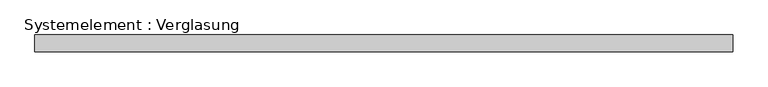
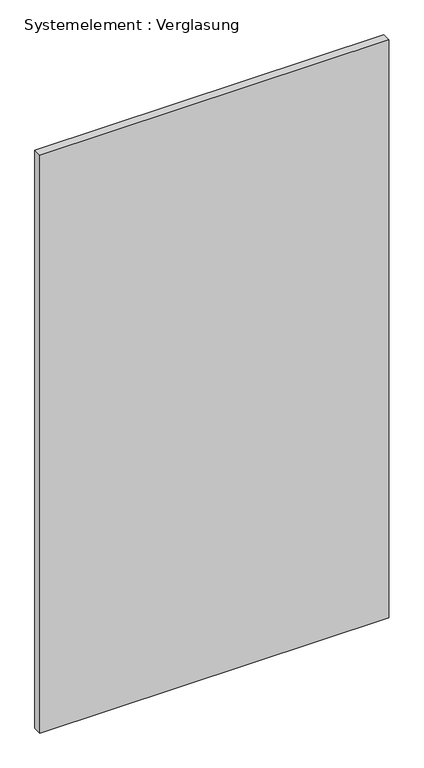
"""IFC4 building model written with IfcOpenShell, lengths in millimetres: plate geometry, Systemelement : Verglasung."""

import ifcopenshell
import ifcopenshell.guid

model = None  # the IFC model being written
_history = None  # IfcOwnerHistory: only IFC2X3 demands one
_inside = {}  # id of a spatial element -> (the spatial element, [elements in it])
_under = {}  # id of a project, library or spatial element -> (it, [spatial elements below it])
_declared = {}  # id of a project -> (the project, [libraries it declares])
_typed = {}  # id of a type object -> (the type object, [elements of that type])
_made_of = {}  # id of a material, layer set ... -> (it, [elements and type objects made of it])


def new_model(schema):
    """Start an empty IFC model of exactly this schema.

    Asked for "IFC4X3", IfcOpenShell would pick the latest addendum, in which some entities
    have other attributes; the version numbers below select the first issue.
    IFC2X3 requires an IfcOwnerHistory on every rooted entity: one is made here for all.
    """
    global model, _history
    if schema == "IFC4X3":
        model = ifcopenshell.file(schema_version=(4, 3, 0, 0))
    else:
        model = ifcopenshell.file(schema=schema)
    _inside.clear()
    _under.clear()
    _declared.clear()
    _typed.clear()
    _made_of.clear()
    _history = None
    if model.schema == "IFC2X3":
        org = make("IfcOrganization", Name="unknown")
        user = make(
            "IfcPersonAndOrganization",
            ThePerson=make("IfcPerson", FamilyName="unknown"),
            TheOrganization=org,
        )
        app = make(
            "IfcApplication",
            ApplicationDeveloper=org,
            Version="unknown",
            ApplicationFullName="unknown",
            ApplicationIdentifier="unknown",
        )
        _history = make(
            "IfcOwnerHistory",
            OwningUser=user,
            OwningApplication=app,
            ChangeAction="ADDED",
            CreationDate=0,
        )
    return model


def make(cls, **values):
    """One entity of the class cls with the attributes given. An attribute that is None is left unset."""
    return model.create_entity(
        cls, **{name: value for name, value in values.items() if value is not None}
    )


def rooted(cls, **values):
    """An entity with a GlobalId (a new one), such as an element, a storey or a relation."""
    return make(cls, GlobalId=ifcopenshell.guid.new(), OwnerHistory=_history, **values)


def si_unit(unit_type, name, prefix=None):
    """IfcSIUnit, for example si_unit("LENGTHUNIT", "METRE", prefix="MILLI")."""
    return make("IfcSIUnit", UnitType=unit_type, Prefix=prefix, Name=name)


def assignment(units):
    """IfcUnitAssignment: the units of a project."""
    return None if units is None else make("IfcUnitAssignment", Units=units)


def point(xyz):
    """IfcCartesianPoint."""
    return None if xyz is None else make("IfcCartesianPoint", Coordinates=xyz)


def direction(xyz):
    """IfcDirection."""
    return None if xyz is None else make("IfcDirection", DirectionRatios=xyz)


def frame(location, z_axis=None, x_axis=None):
    """IfcAxis2Placement3D, a coordinate frame: its origin and axes. An axis left out is left unset."""
    return make(
        "IfcAxis2Placement3D",
        Location=point(location),
        Axis=direction(z_axis),
        RefDirection=direction(x_axis),
    )


def origin():
    """The frame at (0, 0, 0) with its axes left unset."""
    return frame((0.0, 0.0, 0.0))


def origin_with_axes():
    """The frame at (0, 0, 0) with the z axis (0, 0, 1) and the x axis (1, 0, 0) written out."""
    return frame((0.0, 0.0, 0.0), z_axis=(0.0, 0.0, 1.0), x_axis=(1.0, 0.0, 0.0))


def place(relative_to, where):
    """IfcLocalPlacement: puts the frame where relative to a parent placement (None: the world)."""
    return make(
        "IfcLocalPlacement", PlacementRelTo=relative_to, RelativePlacement=where
    )


def context(
    kind, dimensions, precision=None, world=None, true_north=None, identifier=None
):
    """IfcGeometricRepresentationContext, for example the 3D "Model" context."""
    return make(
        "IfcGeometricRepresentationContext",
        ContextIdentifier=identifier,
        ContextType=kind,
        CoordinateSpaceDimension=dimensions,
        Precision=precision,
        WorldCoordinateSystem=world,
        TrueNorth=true_north,
    )


def project(units=None, contexts=None):
    """IfcProject with its units and contexts."""
    return rooted(
        "IfcProject",
        Name="project",
        RepresentationContexts=contexts,
        UnitsInContext=assignment(units),
    )


def spatial(cls, under=None, at=None, **own):
    """A site, building, storey or space (cls), placed at a placement, below another one or the project."""
    s = rooted(cls, ObjectPlacement=at, **own)
    if under is not None:
        _under.setdefault(under.id(), (under, []))[1].append(s)
    return s


def polyline(points):
    """IfcPolyline through the points."""
    return make("IfcPolyline", Points=[point(p) for p in points])


def outline(outer, holes=None, kind="AREA"):
    """IfcArbitraryClosedProfileDef: a profile drawn as a closed curve; with holes, ...WithVoids."""
    if holes is None:
        return make("IfcArbitraryClosedProfileDef", ProfileType=kind, OuterCurve=outer)
    return make(
        "IfcArbitraryProfileDefWithVoids",
        ProfileType=kind,
        OuterCurve=outer,
        InnerCurves=holes,
    )


def extrude(swept, where, along, depth):
    """IfcExtrudedAreaSolid: the profile swept, set in the frame where, extruded along a direction by depth."""
    return make(
        "IfcExtrudedAreaSolid",
        SweptArea=swept,
        Position=where,
        ExtrudedDirection=direction(along),
        Depth=depth,
    )


def shape(context_of_items, identifier, shape_type, items):
    """IfcShapeRepresentation: the items that make up one representation, for example the "Body"."""
    return make(
        "IfcShapeRepresentation",
        ContextOfItems=context_of_items,
        RepresentationIdentifier=identifier,
        RepresentationType=shape_type,
        Items=items,
    )


def source(mapping_origin, context_of_items, identifier, shape_type, items):
    """IfcRepresentationMap: a shape defined once, which mapped items show again and again."""
    return make(
        "IfcRepresentationMap",
        MappingOrigin=mapping_origin,
        MappedRepresentation=shape(context_of_items, identifier, shape_type, items),
    )


def transform(
    local_origin,
    x_axis=None,
    y_axis=None,
    z_axis=None,
    scale=None,
    scale2=None,
    scale3=None,
    uniform=True,
):
    """IfcCartesianTransformationOperator3D, or its non-uniform kind. x_axis, y_axis, z_axis: its Axis1, 2, 3."""
    if uniform:
        return make(
            "IfcCartesianTransformationOperator3D",
            Axis1=direction(x_axis),
            Axis2=direction(y_axis),
            LocalOrigin=point(local_origin),
            Scale=scale,
            Axis3=direction(z_axis),
        )
    return make(
        "IfcCartesianTransformationOperator3DnonUniform",
        Axis1=direction(x_axis),
        Axis2=direction(y_axis),
        LocalOrigin=point(local_origin),
        Scale=scale,
        Axis3=direction(z_axis),
        Scale2=scale2,
        Scale3=scale3,
    )


def mapped(mapping_source, mapping_target):
    """IfcMappedItem: shows the shape of a source again, moved by a transform."""
    return make(
        "IfcMappedItem", MappingSource=mapping_source, MappingTarget=mapping_target
    )


def made_of(thing, what):
    """Note that an element or type object is made of a material, layer set ...; save() writes the relation."""
    if what is not None:
        _made_of.setdefault(what.id(), (what, []))[1].append(thing)
    return thing


def element(
    cls,
    number,
    at=None,
    inside=None,
    cuts=None,
    type_object=None,
    material=None,
    context=None,
    identifier="Body",
    shape_type=None,
    held_by="IfcProductDefinitionShape",
    body=None,
    shapes=None,
    **own,
):
    """One element of the class cls, such as IfcWall. Its Tag is "e" and its number.

    at: its placement. inside: the storey or other place that contains it. cuts: it is an
    opening in that element (IfcRelVoidsElement). A single representation is given by context,
    identifier, shape_type and body (its items); several are given by shapes. held_by: the class
    of the entity that holds the representations. save() writes the other relations.
    """
    e = rooted(cls, Tag="e%d" % number, ObjectPlacement=at, **own)
    if body is not None:
        shapes = [shape(context, identifier, shape_type, body)]
    if shapes is not None:
        e.Representation = make(held_by, Representations=shapes)
    if inside is not None:
        _inside.setdefault(inside.id(), (inside, []))[1].append(e)
    if cuts is not None:
        rooted(
            "IfcRelVoidsElement", RelatingBuildingElement=cuts, RelatedOpeningElement=e
        )
    if type_object is not None:
        _typed.setdefault(type_object.id(), (type_object, []))[1].append(e)
    return made_of(e, material)


def aggregate(whole, parts):
    """IfcRelAggregates: a whole, such as a stair, and the parts it consists of."""
    return rooted("IfcRelAggregates", RelatingObject=whole, RelatedObjects=parts)


def save(model, path):
    """Write the relations noted so far, then the file.

    IfcRelAggregates (storeys below a building ...), IfcRelContainedInSpatialStructure (elements
    in a storey), IfcRelDefinesByType, IfcRelAssociatesMaterial and IfcRelDeclares: one each for
    every whole, place, type object, material and project.
    """
    for whole, parts in _under.values():
        aggregate(whole, parts)
    for where, things in _inside.values():
        rooted(
            "IfcRelContainedInSpatialStructure",
            RelatedElements=things,
            RelatingStructure=where,
        )
    for kind, things in _typed.values():
        rooted("IfcRelDefinesByType", RelatedObjects=things, RelatingType=kind)
    for what, things in _made_of.values():
        rooted("IfcRelAssociatesMaterial", RelatedObjects=things, RelatingMaterial=what)
    for by, libraries in _declared.values():
        rooted("IfcRelDeclares", RelatingContext=by, RelatedDefinitions=libraries)
    model.write(path)


def systemelement_verglasung_38ed9cad(model_context):
    return source(origin(), model_context, "Body", "SweptSolid", [
        extrude(outline(polyline([(620.0, -15.0), (-620.0, -15.0), (-620.0, 15.0), (620.0, 15.0), (620.0, -15.0)])), origin_with_axes(), (0.0, 0.0, 1.0), 2170.8558388),
    ])


if __name__ == "__main__":
    model = new_model("IFC4")
    model_context = context("Model", 3, world=origin())
    ifc_project = project(units=[si_unit("LENGTHUNIT", "METRE", prefix="MILLI")], contexts=[model_context])
    site = spatial("IfcSite", under=ifc_project)
    building = spatial("IfcBuilding", under=site)
    placement = place(None, origin())
    systemelement_verglasung_shape = systemelement_verglasung_38ed9cad(model_context)
    element("IfcPlate", 1, ObjectType="Systemelement : Verglasung", at=placement, inside=building, context=model_context, shape_type="MappedRepresentation", body=[
        mapped(systemelement_verglasung_shape, transform((0.0, 0.0, 0.0), x_axis=(1.0, 0.0, 0.0), y_axis=(0.0, 1.0, 0.0), z_axis=(0.0, 0.0, 1.0))),
    ])
    save(model, "model.ifc")

# Revit data of these elements
# Type "Systemelement : Verglasung"
#   Construction Type Id = "GSP4R"
#   Analytic Construction = "1/8 Zoll Pilkington-Verglasung einfach"
#   Visual Light Transmittance = 0.9
#   Solar Heat Gain Coefficient = 0.86
#   Heat Transfer Coefficient (U) = 6.7069 W/(m²·K)
# Element 1 (IfcPlate, "Systemelement : Verglasung")
#   Materials on its faces: "Glas"
# Materials
#   "Glas": class "Glas", colour RGB 0 0 255, transparency 0.75, Comments = "Render-Darstellung nicht aktualisiert ", Cost = 0
